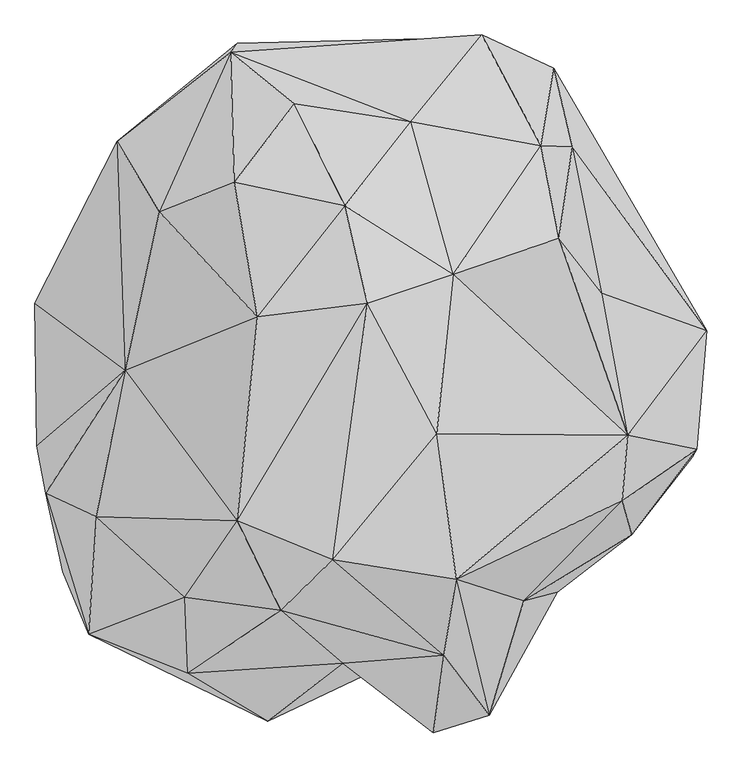
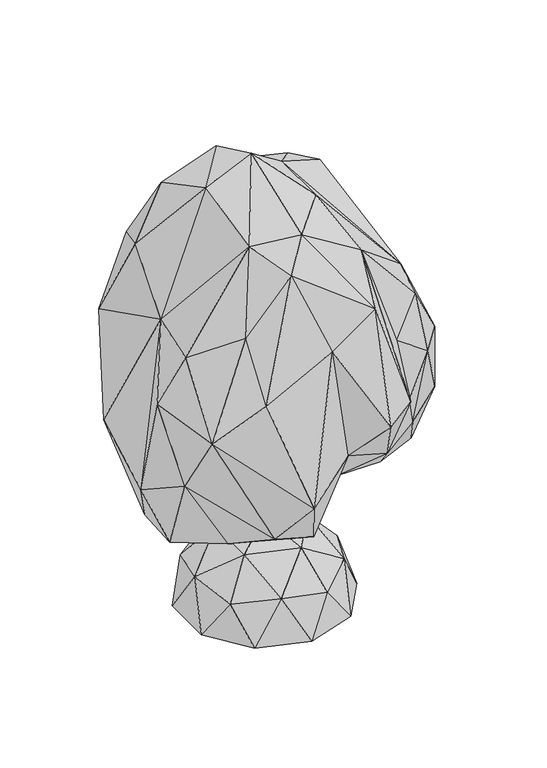
"""IFC4 building model written with IfcOpenShell, lengths in millimetres: geographic element geometry, Enscape AssetDefinition - Evergreen Tree 026 Mangrove Tree : Enscape AssetDefinition - Evergreen Tree 026 Mangrove Tree."""

from ifc_helpers import new_model, si_unit, origin, place, context, project, spatial, faceted_brep, source, transform, mapped, element, save


def geographic_element_ad668b55(model_context):
    return source(origin(), model_context, "Body", "Brep", [
        faceted_brep([(759.3850493, 2155.7788849, 3421.6880798), (857.2466373, 2173.4480858, 4260.392189), (1310.6087446, 1963.4292126, 3645.2572346), (1229.2288542, 1477.4450064, 5251.5659332), (412.5328064, 1626.1132956, 5345.2262878), (-721.0861444, 2063.5442734, 4396.9154358), (1427.7268648, 1471.421957, 4610.6462479), (677.223742, 669.5683002, 5807.4908257), (1343.3746099, 894.6408629, 5465.3263092), (-4.6136379, 1098.0086327, 6018.1393623), (-319.5822239, 1739.5195961, 5225.2759933), (138.4629309, 487.2009456, 6229.7720909), (575.8342743, -333.5238695, 5951.672554), (1775.5553722, -343.6187208, 4506.3047409), (1612.9266024, 548.2248068, 4613.6369705), (1741.7427301, -756.1084628, 4314.6924973), (696.2387562, -1248.1001616, 5640.1820183), (2209.3684673, -430.9785664, 3466.4051533), (2273.3225822, 313.4104908, 3308.0215454), (-78.1980827, -1127.7376413, 6062.1490479), (-680.3830266, -882.2895288, 5943.9444542), (-406.1282873, -1443.385005, 5756.3405037), (619.6721196, -1728.1042337, 5073.5721588), (-990.9824133, -1841.3853645, 4246.6049194), (-16.8974381, -1776.1263847, 4680.4294586), (-1009.7441673, -1363.0107641, 4982.1333885), (904.8481584, -2105.2441597, 3809.4029427), (552.8903008, -2215.4510021, 3615.8227921), (-488.3022904, -2141.8128014, 2718.4286118), (176.066488, -1826.7502785, 3083.1065178), (-1614.6217585, -1596.0488319, 3746.8745708), (-1565.190196, -856.3057184, 4577.0697594), (-856.1306596, -1816.6046143, 2191.9298172), (-1777.1856785, -1202.4165392, 2938.0102158), (-1885.0727081, -708.6624503, 3904.415369), (-292.4755216, -1799.6582985, 2021.6724873), (-1139.3172741, -1152.8451443, 1823.4864473), (-1690.730691, -680.9649467, 1753.0386448), (-1941.7048693, -410.2519155, 2461.1241817), (-1384.2458725, 66.2233606, 4528.2020569), (-1951.8153667, 487.8905118, 2966.5203094), (-1435.1681471, 1505.0789118, 3834.31077), (-552.3230433, 400.652945, 6007.7409744), (-1169.9451208, 1062.4083281, 4984.7383499), (-1679.1715622, -54.3161258, 1778.3066034), (-1119.7994947, 607.5105667, 2237.916708), (-1029.7919512, 1378.1731129, 2421.5624332), (-1441.1090612, 1242.9260015, 3036.8125439), (-1065.2612448, -253.0918419, 1429.0599823), (-1031.0028791, 241.449669, 1833.4736824), (-578.3851147, 808.3070517, 2094.7737694), (781.6776037, 1889.4867897, 2201.4584541), (-803.2484055, 1888.7063265, 3013.2524967), (-678.067863, 2120.9189892, 3801.7504215), (1208.4562778, 1806.8442345, 2868.516922), (1306.2992096, 817.6057339, 2028.1648636), (-698.1117725, 1245.9238768, 5622.5824356), (2141.6327953, 310.4840517, 2196.0556507), (2181.6756725, -480.9265435, 2608.9737415), (1530.2058458, -1068.1143999, 2664.2003059), (1898.4498978, -397.7695405, 1883.5673332), (1800.0426292, -969.1437483, 3569.4565773), (1122.7493286, -1384.5052719, 4216.3152695), (1331.8195343, -1329.7909498, 3218.1782722), (697.3488927, -1887.7682686, 2980.4532528), (547.5997925, -900.7822871, 2098.8767147), (482.2958708, -597.7678299, 1936.1444712), (1541.2700176, -250.7503033, 1564.1474724), (-576.639235, -1001.2054443, 1725.8800268), (-381.8668127, 152.5972784, 2235.1076603), (430.0787151, 280.9780836, 2048.6762524), (1182.5038195, -8.4966449, 1575.804472)], [[[0, 1, 2]], [[1, 3, 2]], [[1, 4, 3]], [[1, 5, 4]], [[1, 0, 5]], [[2, 3, 6]], [[7, 8, 3]], [[8, 6, 3]], [[4, 7, 3]], [[9, 7, 4]], [[10, 9, 4]], [[4, 5, 10]], [[11, 7, 9]], [[12, 7, 11]], [[7, 12, 13]], [[7, 13, 8]], [[14, 6, 8]], [[13, 14, 8]], [[15, 13, 16]], [[16, 13, 12]], [[17, 13, 15]], [[18, 13, 17]], [[14, 13, 18]], [[19, 16, 12]], [[12, 11, 19]], [[20, 21, 19]], [[19, 22, 16]], [[20, 19, 11]], [[19, 21, 22]], [[23, 24, 21]], [[20, 25, 21]], [[24, 22, 21]], [[23, 21, 25]], [[26, 16, 22]], [[27, 26, 22]], [[27, 22, 24]], [[28, 29, 24]], [[28, 24, 23]], [[29, 27, 24]], [[28, 23, 30]], [[23, 25, 30]], [[20, 31, 25]], [[30, 25, 31]], [[32, 30, 33]], [[33, 30, 34]], [[31, 34, 30]], [[32, 28, 30]], [[32, 35, 28]], [[35, 29, 28]], [[36, 32, 33]], [[35, 32, 36]], [[37, 36, 33]], [[37, 33, 38]], [[33, 34, 38]], [[31, 39, 34]], [[39, 38, 34]], [[31, 20, 39]], [[40, 39, 41]], [[42, 43, 39]], [[40, 38, 39]], [[39, 43, 41]], [[20, 42, 39]], [[40, 44, 38]], [[38, 44, 37]], [[44, 40, 45]], [[46, 45, 40]], [[40, 47, 46]], [[47, 40, 41]], [[44, 48, 37]], [[48, 44, 49]], [[44, 45, 49]], [[46, 50, 45]], [[49, 45, 50]], [[51, 46, 52]], [[47, 52, 46]], [[46, 51, 50]], [[41, 52, 47]], [[53, 0, 52]], [[53, 52, 41]], [[52, 0, 51]], [[51, 0, 54]], [[50, 51, 55]], [[54, 55, 51]], [[2, 54, 0]], [[5, 0, 53]], [[41, 5, 53]], [[43, 5, 41]], [[43, 56, 5]], [[56, 10, 5]], [[42, 56, 43]], [[9, 10, 56]], [[56, 42, 9]], [[9, 42, 11]], [[20, 11, 42]], [[2, 6, 18]], [[57, 2, 18]], [[54, 2, 57]], [[18, 6, 14]], [[18, 58, 57]], [[17, 58, 18]], [[59, 60, 58]], [[60, 57, 58]], [[58, 17, 61]], [[58, 61, 59]], [[61, 17, 15]], [[61, 15, 62]], [[63, 61, 62]], [[63, 59, 61]], [[62, 15, 16]], [[26, 62, 16]], [[26, 63, 62]], [[26, 64, 63]], [[59, 63, 64]], [[27, 64, 26]], [[65, 64, 29]], [[29, 64, 27]], [[64, 65, 59]], [[35, 65, 29]], [[65, 66, 67]], [[67, 59, 65]], [[35, 68, 65]], [[66, 65, 68]], [[36, 68, 35]], [[68, 69, 66]], [[48, 68, 36]], [[68, 48, 69]], [[37, 48, 36]], [[69, 48, 49]], [[50, 70, 69]], [[49, 50, 69]], [[66, 69, 70]], [[70, 55, 71]], [[70, 71, 66]], [[50, 55, 70]], [[54, 57, 55]], [[67, 55, 57]], [[55, 67, 71]], [[71, 67, 66]], [[67, 57, 60]], [[67, 60, 59]]]),
        faceted_brep([(95.4975113, -55.1357642, 2234.1609001), (95.4975113, 55.1357642, 0.0), (95.4975113, 55.1357642, 2234.1609001), (95.4975113, -55.1357642, 0.0), (0.0, 110.2705523, 0.0), (-95.4975113, -55.1357642, 0.0), (0.0, 110.2705523, 2234.1609001), (0.0, -110.2705523, 2234.1609001), (0.0, -110.2705523, 0.0), (-95.4975113, -55.1357642, 2234.1609001), (-95.4975113, 55.1357642, 2234.1609001), (-95.4975113, 55.1357642, 0.0)], [[[0, 1, 2]], [[3, 1, 0]], [[1, 4, 2]], [[1, 5, 4]], [[3, 5, 1]], [[2, 4, 6]], [[6, 0, 2]], [[7, 3, 0]], [[0, 6, 7]], [[8, 3, 7]], [[5, 3, 8]], [[5, 8, 9]], [[10, 5, 9]], [[11, 5, 10]], [[4, 5, 11]], [[4, 11, 6]], [[6, 11, 10]], [[9, 6, 10]], [[7, 6, 9]], [[9, 8, 7]]]),
        faceted_brep([(256.5885186, -535.8294845, 897.5829482), (388.3896768, -941.4785504, 430.8758378), (864.7769094, -535.8314514, 521.7059255), (-235.442251, -893.3106661, 521.7078924), (68.6539114, -1114.2526865, -86.4844397), (748.6261129, -893.3165669, -86.4844397), (68.6539114, 42.5829887, 1070.3513622), (-423.3748913, -314.892292, 897.5829482), (676.8374443, 42.5829887, 897.5800276), (-768.4412003, -565.5946732, 430.8748841), (-611.3182902, -893.3165669, -86.4844397), (748.6261129, 978.4834385, -86.4844397), (1168.872118, -314.8932755, -86.4844397), (1103.3588648, 42.5829887, 430.87098), (1168.872118, 400.0602067, -86.4844397), (864.7769094, 620.9984422, 521.7059255), (256.5885186, 620.9964752, 897.5829482), (388.3896768, 1026.6455412, 430.8758378), (-235.442251, 978.4775972, 521.7078924), (-423.3748913, 400.059253, 897.5829482), (68.6539114, 1199.4196177, -86.4844397), (-768.4412003, 650.7616639, 430.8748841), (-611.3182902, 978.4834385, -86.4844397), (-915.4066443, 42.5829887, 521.7059255), (-1031.5642357, 400.0602067, -86.4844397), (-1031.5642357, -314.8932755, -86.4844397)], [[[0, 1, 2]], [[0, 3, 1]], [[3, 4, 1]], [[1, 5, 2]], [[1, 4, 5]], [[6, 7, 0]], [[0, 7, 3]], [[6, 0, 8]], [[8, 0, 2]], [[7, 9, 3]], [[9, 10, 3]], [[3, 10, 4]], [[4, 11, 5]], [[10, 11, 4]], [[2, 5, 12]], [[5, 11, 12]], [[2, 12, 13]], [[13, 12, 14]], [[12, 11, 14]], [[8, 13, 15]], [[8, 2, 13]], [[13, 14, 15]], [[15, 14, 11]], [[16, 8, 15]], [[16, 15, 17]], [[15, 11, 17]], [[16, 17, 18]], [[6, 8, 16]], [[6, 16, 19]], [[19, 16, 18]], [[17, 20, 18]], [[17, 11, 20]], [[19, 18, 21]], [[18, 20, 22]], [[18, 22, 21]], [[19, 21, 23]], [[6, 19, 7]], [[7, 19, 23]], [[21, 24, 23]], [[21, 22, 24]], [[22, 11, 24]], [[11, 22, 20]], [[23, 24, 25]], [[24, 11, 25]], [[7, 23, 9]], [[23, 25, 9]], [[9, 25, 10]], [[25, 11, 10]]]),
    ])


if __name__ == "__main__":
    model = new_model("IFC4")
    model_context = context("Model", 3, world=origin())
    ifc_project = project(units=[si_unit("LENGTHUNIT", "METRE", prefix="MILLI")], contexts=[model_context])
    site = spatial("IfcSite", under=ifc_project)
    building = spatial("IfcBuilding", under=site)
    placement = place(None, origin())
    geographic_element_shape = geographic_element_ad668b55(model_context)
    element("IfcGeographicElement", 1, ObjectType="Enscape AssetDefinition - Evergreen Tree 026 Mangrove Tree : Enscape AssetDefinition - Evergreen Tree 026 Mangrove Tree", at=placement, inside=building, context=model_context, shape_type="MappedRepresentation", body=[
        mapped(geographic_element_shape, transform((0.0, 0.0, 0.0), x_axis=(1.0, 0.0, 0.0), y_axis=(0.0, 1.0, 0.0), z_axis=(0.0, 0.0, 1.0))),
    ])
    save(model, "model.ifc")

# Revit data of these elements
# Type "Enscape AssetDefinition - Evergreen Tree 026 Mangrove Tree : Enscape AssetDefinition - Evergreen Tree 026 Mangrove Tree"
#   EnscapeAssetSource = "REMOTE"
#   EnscapeAssetId = "a65c7032-a677-49d1-8808-0d12866f0340"
#   Height = 6.229772 m
#   EnscapeNativeAssetHeight = 6.229772 m
#   Default Elevation = 0
